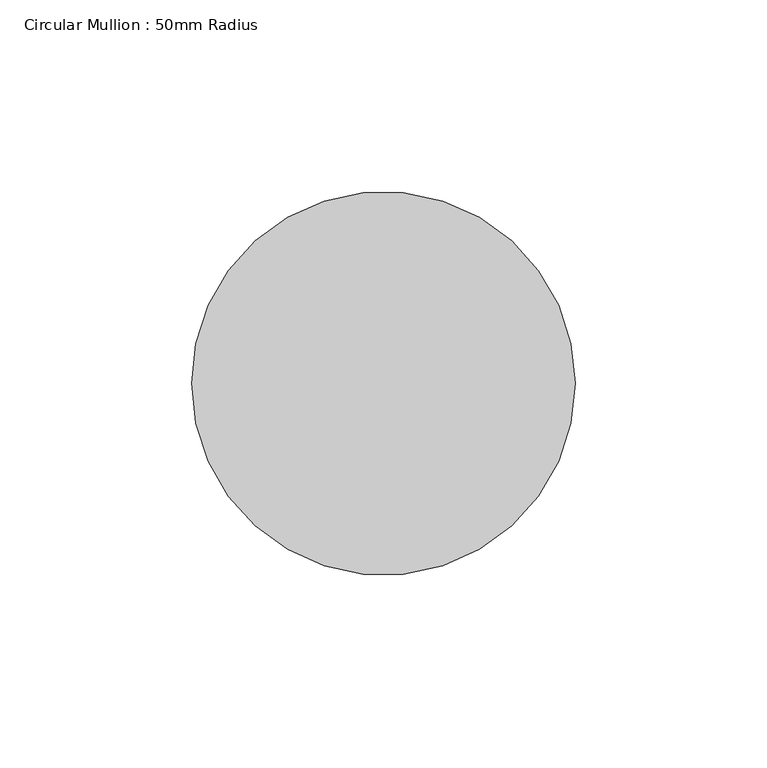
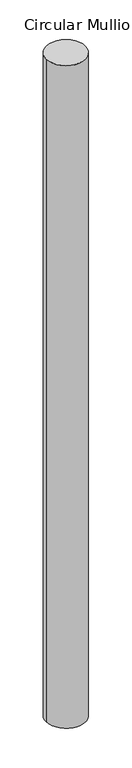
"""IFC4 building model written with IfcOpenShell, lengths in millimetres: member geometry, Circular Mullion : 50mm Radius."""

from ifc_helpers import new_model, si_unit, point, frame, origin, origin_2d, place, context, project, spatial, circle_curve, trimmed, segment, composite_curve, outline, extrude, source, transform, mapped, element, save


def circular_mullion_50mm_radius_0a7a2059(model_context):
    return source(origin(), model_context, "Body", "SweptSolid", [
        extrude(outline(composite_curve([segment(trimmed(circle_curve(origin_2d(), 50.0), [point((50.0, 0.0))], [point((-50.0, 0.0))], False, "CARTESIAN"), True, "CONTINUOUS"), segment(trimmed(circle_curve(origin_2d(), 50.0), [point((-50.0, 0.0))], [point((50.0, 0.0))], False, "CARTESIAN"), True, "CONTINUOUS")], self_intersect=False)), frame((0.0, 0.0, -1786.6827336), z_axis=(0.0, 0.0, 1.0), x_axis=(1.0, 0.0, 0.0)), (0.0, 0.0, 1.0), 1786.6827336),
    ])


if __name__ == "__main__":
    model = new_model("IFC4")
    model_context = context("Model", 3, world=origin())
    ifc_project = project(units=[si_unit("LENGTHUNIT", "METRE", prefix="MILLI")], contexts=[model_context])
    site = spatial("IfcSite", under=ifc_project)
    building = spatial("IfcBuilding", under=site)
    placement = place(None, origin())
    circular_mullion_50mm_radius_shape = circular_mullion_50mm_radius_0a7a2059(model_context)
    element("IfcMember", 1, ObjectType="Circular Mullion : 50mm Radius", at=placement, inside=building, context=model_context, shape_type="MappedRepresentation", body=[
        mapped(circular_mullion_50mm_radius_shape, transform((0.0, 0.0, 0.0), x_axis=(1.0, 0.0, 0.0), y_axis=(0.0, 1.0, 0.0), z_axis=(0.0, 0.0, 1.0))),
    ])
    save(model, "model.ifc")

# Revit data of these elements
# Type "Circular Mullion : 50mm Radius"
#   built-in parameter 1007350 = 0.164042 (stored number, unit not read)
# Element 1 (IfcMember, "Circular Mullion : 50mm Radius")
#   Materials on its faces: "Aluminium"
# Materials
#   "Aluminium": class "Metal", colour RGB 247 247 247, transparency 0, Description = "Aluminium 6061", Cost = 0
